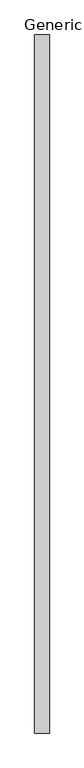
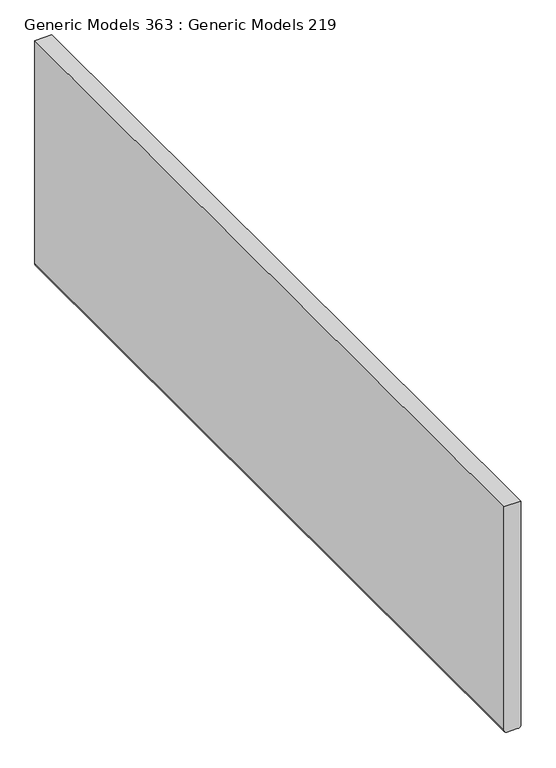
"""IFC4 building model written with IfcOpenShell, lengths in millimetres: proxy geometry, Generic Models 363 : Generic Models 219."""

from ifc_helpers import new_model, si_unit, point, frame, frame_2d, origin, place, context, project, spatial, polyline, circle_curve, trimmed, segment, composite_curve, outline, extrude, source, transform, mapped, element, save


def generic_models_363_generic_models_219_e38cb05f(model_context):
    return source(origin(), model_context, "Body", "SweptSolid", [
        extrude(outline(composite_curve([segment(polyline([(127414.9852, -6852.0116813), (128116.9606599, -6852.0116813), (128116.9606599, -6902.8116813), (127414.9852, -6902.8116813)]), True, "CONTINUOUS"), segment(trimmed(circle_curve(frame_2d((127414.9852, -6893.9724813)), 8.8392), [point((127414.9852, -6902.8116813))], [point((127406.146, -6893.9724813))], False, "CARTESIAN"), True, "CONTINUOUS"), segment(polyline([(127406.146, -6893.9724813), (127406.146, -6860.8508813)]), True, "CONTINUOUS"), segment(trimmed(circle_curve(frame_2d((127414.9852, -6860.8508813)), 8.8392), [point((127406.146, -6860.8508813))], [point((127414.9852, -6852.0116813))], False, "CARTESIAN"), True, "CONTINUOUS")], self_intersect=False)), frame((0.0, -5782.2723769, 0.0), z_axis=(0.0, 1.0, 0.0), x_axis=(0.0, 0.0, 1.0)), (0.0, 0.0, 1.0), 2417.6222388),
    ])


if __name__ == "__main__":
    model = new_model("IFC4")
    model_context = context("Model", 3, world=origin())
    ifc_project = project(units=[si_unit("LENGTHUNIT", "METRE", prefix="MILLI")], contexts=[model_context])
    site = spatial("IfcSite", under=ifc_project)
    building = spatial("IfcBuilding", under=site)
    placement = place(None, origin())
    generic_models_363_generic_models_219_shape = generic_models_363_generic_models_219_e38cb05f(model_context)
    element("IfcBuildingElementProxy", 1, Name="Generic Models 363 : Generic Models 219", ObjectType="Generic Models 363 : Generic Models 219", at=placement, inside=building, context=model_context, shape_type="MappedRepresentation", body=[
        mapped(generic_models_363_generic_models_219_shape, transform((0.0, 0.0, 0.0), x_axis=(1.0, 0.0, 0.0), y_axis=(0.0, 1.0, 0.0), z_axis=(0.0, 0.0, 1.0))),
    ])
    save(model, "model.ifc")

# Revit data of these elements
# Element 1 (IfcBuildingElementProxy, "Generic Models 363 : Generic Models 219")
#   Materials on its faces: "_PLANTATION STYLE SHUTTERS BY OWNER"
# Materials
#   "_PLANTATION STYLE SHUTTERS BY OWNER": class "Metal", colour RGB 209 202 188, transparency 0, Description = "Structural steel 50ksi", Cost = 0
